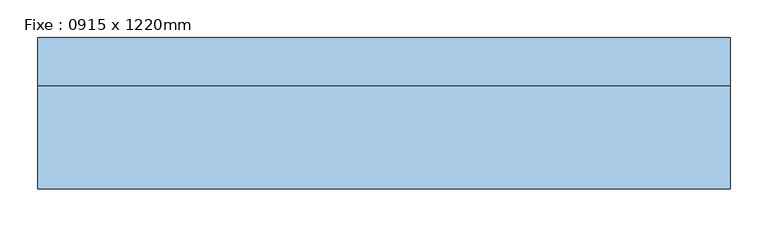
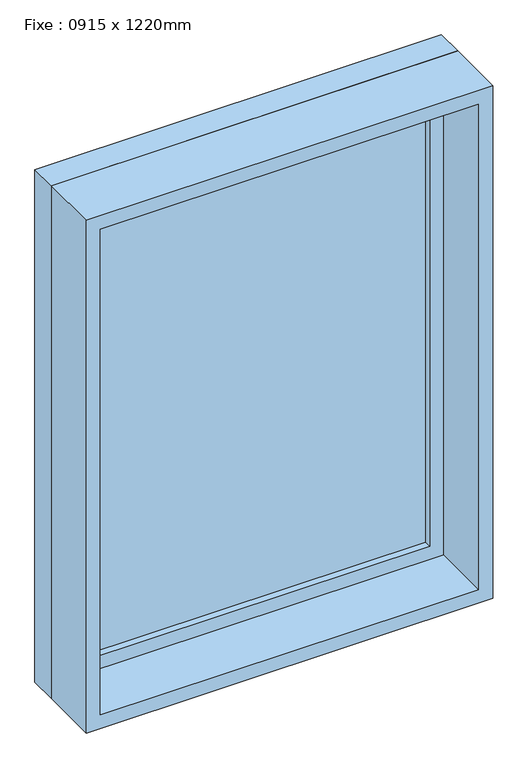
"""IFC4 building model written with IfcOpenShell, lengths in millimetres: window geometry, Fixe : 0915 x 1220mm."""

from ifc_helpers import new_model, si_unit, frame, origin, place, context, project, spatial, polyline, outline, extrude, source, transform, mapped, element, save


def fixe_0915_x_1220mm_488fb2fb(model_context):
    return source(origin(), model_context, "Body", "SweptSolid", [
        extrude(outline(polyline([(-394.5, 78.0), (394.5, 78.0), (394.5, 66.0), (-394.5, 66.0), (-394.5, 78.0)])), frame((0.0, 0.0, 978.0), z_axis=(0.0, 0.0, 1.0), x_axis=(1.0, 0.0, 0.0)), (0.0, 0.0, 1.0), 1094.0),
        extrude(outline(polyline([(2116.0, -438.5), (934.0, -438.5), (934.0, 438.5), (2116.0, 438.5), (2116.0, -438.5)]), holes=[polyline([(2072.0, -394.5), (2072.0, 394.5), (978.0, 394.5), (978.0, -394.5), (2072.0, -394.5)])]), frame((0.0, 50.0, 0.0), z_axis=(0.0, 1.0, 0.0), x_axis=(0.0, 0.0, 1.0)), (0.0, 0.0, 1.0), 44.0),
        extrude(outline(polyline([(2135.0, -457.5), (915.0, -457.5), (915.0, 457.5), (2135.0, 457.5), (2135.0, -457.5)]), holes=[polyline([(2116.0, -438.5), (2116.0, 438.5), (934.0, 438.5), (934.0, -438.5), (2116.0, -438.5)])]), frame((0.0, 50.0, 0.0), z_axis=(0.0, 1.0, 0.0), x_axis=(0.0, 0.0, 1.0)), (0.0, 0.0, 1.0), 63.0),
        extrude(outline(polyline([(2135.0, -457.5), (915.0, -457.5), (915.0, 457.5), (2135.0, 457.5), (2135.0, -457.5)]), holes=[polyline([(2103.0, -425.5), (2103.0, 425.5), (947.0, 425.5), (947.0, -425.5), (2103.0, -425.5)])]), frame((0.0, -87.0, 0.0), z_axis=(0.0, 1.0, 0.0), x_axis=(0.0, 0.0, 1.0)), (0.0, 0.0, 1.0), 137.0),
    ])


if __name__ == "__main__":
    model = new_model("IFC4")
    model_context = context("Model", 3, world=origin())
    ifc_project = project(units=[si_unit("LENGTHUNIT", "METRE", prefix="MILLI")], contexts=[model_context])
    site = spatial("IfcSite", under=ifc_project)
    building = spatial("IfcBuilding", under=site)
    placement = place(None, origin())
    fixe_0915_x_1220mm_shape = fixe_0915_x_1220mm_488fb2fb(model_context)
    element("IfcWindow", 1, ObjectType="Fixe : 0915 x 1220mm", at=placement, inside=building, context=model_context, shape_type="MappedRepresentation", body=[
        mapped(fixe_0915_x_1220mm_shape, transform((0.0, 0.0, 0.0), x_axis=(1.0, 0.0, 0.0), y_axis=(0.0, 1.0, 0.0), z_axis=(0.0, 0.0, 1.0))),
    ])
    save(model, "model.ifc")

# Revit data of these elements
# Type "Fixe : 0915 x 1220mm"
#   Type Mark = "15"
#   Construction Type Id = "GSP4R"
#   Analytic Construction = "Simple vitrage Pilkington 1/8 po."
#   Visual Light Transmittance = 0.9
#   Solar Heat Gain Coefficient = 0.78
#   Heat Transfer Coefficient (U) = 3.6886 W/(m²·K)
#   Height = 1.22 m
#   Hauteur de l'appui par défaut = 0.915 m
#   Width = 0.915 m
#   Encastrement de fenêtre = 0.019 m
#   Define Thermal Properties by = 1
#   Matériau de cadre extérieur = Châssis
#   Matériau du cadre intérieur = Châssis
#   Matériau du panneau de verre = Verre
#   Châssis = Châssis
#   Wall Closure = (empty or 0)
# Element 1 (IfcWindow, "Fixe : 0915 x 1220mm")
#   Materials on its faces: "Châssis", "Verre"
# Materials
#   "Châssis": class "Bois", colour RGB 224 178 126, transparency 0, Cost = 0
#   "Verre": class "Verre", colour RGB 0 128 192, transparency 0.9, Description = "Verre sodocalcique", Cost = 0
